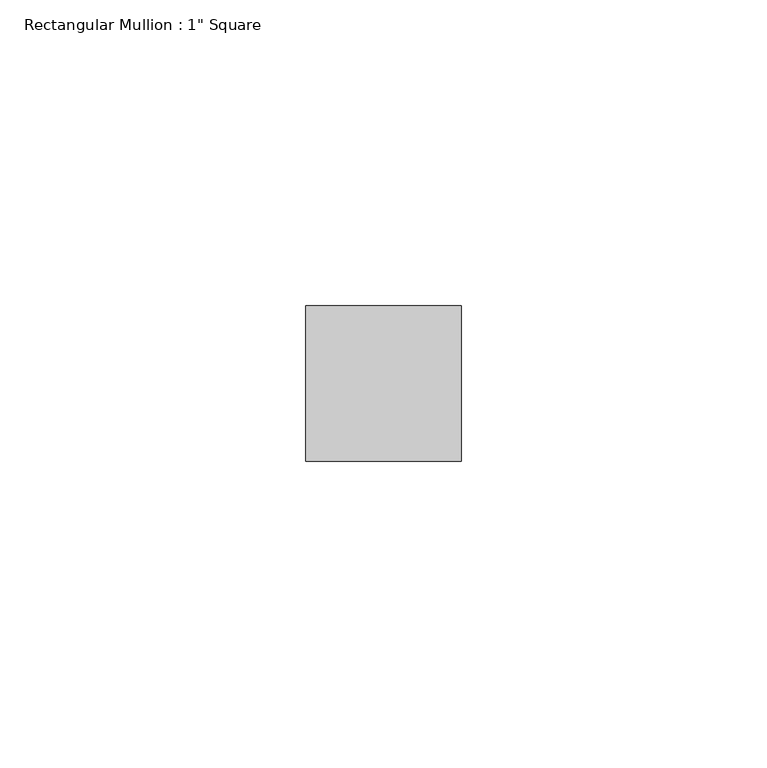
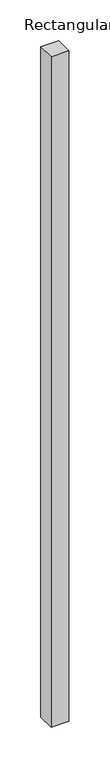
"""IFC4 building model written with IfcOpenShell, lengths in millimetres: member geometry."""

from ifc_helpers import new_model, si_unit, frame, origin, place, context, project, spatial, polyline, outline, extrude, source, transform, mapped, element, save


def member_e449fce7(model_context):
    return source(origin(), model_context, "Body", "SweptSolid", [
        extrude(outline(polyline([(0.0, 12.7), (0.0, -12.7), (-25.4, -12.7), (-25.4, 12.7), (0.0, 12.7)])), frame((0.0, 0.0, -1004.9287927), z_axis=(0.0, 0.0, 1.0), x_axis=(1.0, 0.0, 0.0)), (0.0, 0.0, 1.0), 1004.9287927),
    ])


if __name__ == "__main__":
    model = new_model("IFC4")
    model_context = context("Model", 3, world=origin())
    ifc_project = project(units=[si_unit("LENGTHUNIT", "METRE", prefix="MILLI")], contexts=[model_context])
    site = spatial("IfcSite", under=ifc_project)
    building = spatial("IfcBuilding", under=site)
    placement = place(None, origin())
    member_shape = member_e449fce7(model_context)
    element("IfcMember", 1, ObjectType="Rectangular Mullion : 1\" Square", at=placement, inside=building, context=model_context, shape_type="MappedRepresentation", body=[
        mapped(member_shape, transform((0.0, 0.0, 0.0), x_axis=(1.0, 0.0, 0.0), y_axis=(0.0, 1.0, 0.0), z_axis=(0.0, 0.0, 1.0))),
    ])
    save(model, "model.ifc")

# Revit data of these elements
# Type "Rectangular Mullion : 1\" Square"
#   built-in parameter 1007304 = 0.0833333 (stored number, unit not read)
#   built-in parameter 1007301 = 0.0416667 (stored number, unit not read)
#   built-in parameter 1007300 = 0.0416667 (stored number, unit not read)
# Element 1 (IfcMember, "Rectangular Mullion : 1\" Square")
#   Materials on its faces: "Metal - Aluminum"
# Materials
#   "Metal - Aluminum": class "Metal", colour RGB 247 247 247, transparency 0
